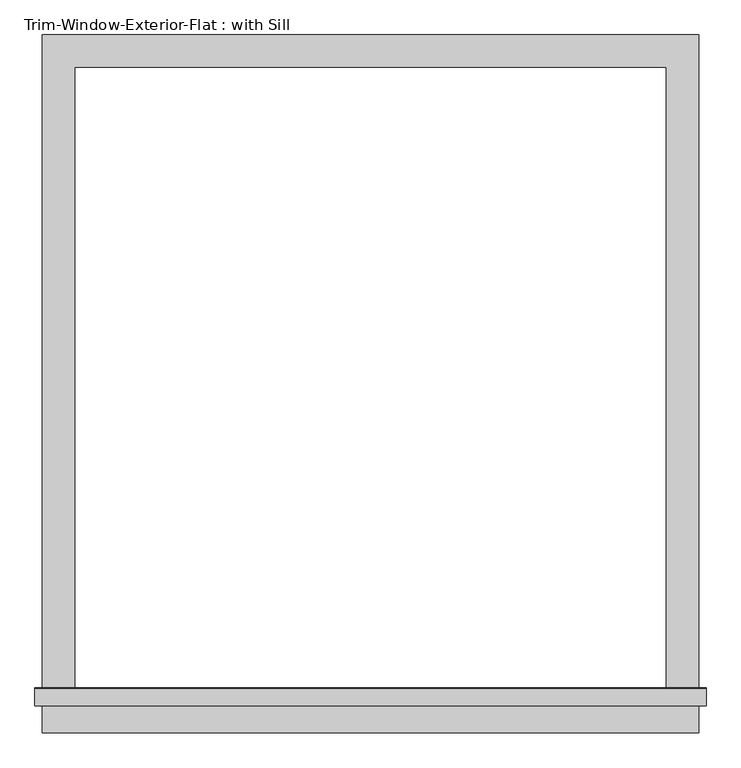
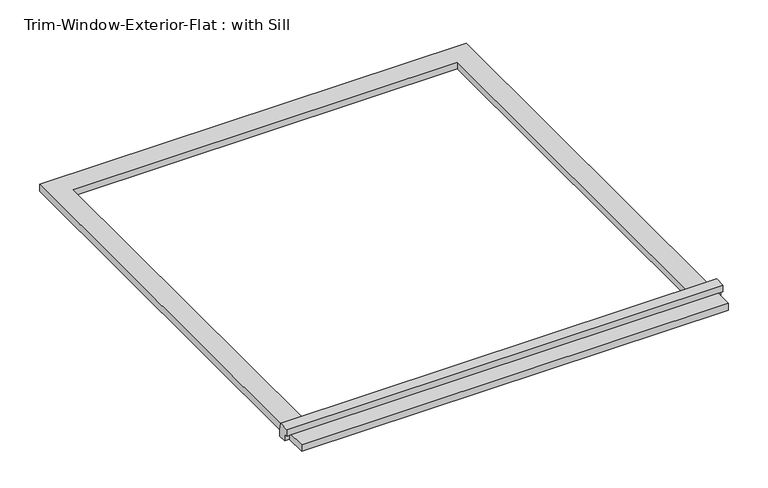
"""IFC4 building model written with IfcOpenShell, lengths in millimetres: proxy geometry, Trim-Window-Exterior-Flat : with Sill."""

from ifc_helpers import new_model, si_unit, frame, origin, origin_with_axes, place, context, project, spatial, polyline, outline, extrude, source, transform, mapped, element, save


def trim_window_exterior_flat_with_sill_d43e16eb(model_context):
    return source(origin(), model_context, "Body", "SweptSolid", [
        extrude(outline(polyline([(577.85, -1114.3823709), (577.85, -1171.5323709), (-577.85, -1171.5323709), (-577.85, -1114.3823709), (577.85, -1114.3823709)])), origin_with_axes(), (0.0, 0.0, 1.0), 19.05),
        extrude(outline(polyline([(-1123.95, 38.1), (-1094.6580645, 38.1), (-1092.2, 19.05), (-1092.2, 0.0), (-1114.3823709, 0.0), (-1114.3823709, 19.05), (-1123.95, 19.05), (-1123.95, 38.1)])), frame((-590.55, 0.0, 0.0), z_axis=(1.0, 0.0, 0.0), x_axis=(0.0, 1.0, 0.0)), (0.0, 0.0, 1.0), 1181.1),
        extrude(outline(polyline([(-577.85, 57.15), (577.85, 57.15), (577.85, -1092.2), (520.7, -1092.2), (520.7, 0.0), (-520.7, 0.0), (-520.7, -1092.2), (-577.85, -1092.2), (-577.85, 57.15)])), origin_with_axes(), (0.0, 0.0, 1.0), 19.05),
    ])


if __name__ == "__main__":
    model = new_model("IFC4")
    model_context = context("Model", 3, world=origin())
    ifc_project = project(units=[si_unit("LENGTHUNIT", "METRE", prefix="MILLI")], contexts=[model_context])
    site = spatial("IfcSite", under=ifc_project)
    building = spatial("IfcBuilding", under=site)
    placement = place(None, origin())
    trim_window_exterior_flat_with_sill_shape = trim_window_exterior_flat_with_sill_d43e16eb(model_context)
    element("IfcBuildingElementProxy", 1, Name="Trim-Window-Exterior-Flat : with Sill", ObjectType="Trim-Window-Exterior-Flat : with Sill", at=placement, inside=building, context=model_context, shape_type="MappedRepresentation", body=[
        mapped(trim_window_exterior_flat_with_sill_shape, transform((0.0, 0.0, 0.0), x_axis=(1.0, 0.0, 0.0), y_axis=(0.0, 1.0, 0.0), z_axis=(0.0, 0.0, 1.0))),
    ])
    save(model, "model.ifc")

# Revit data of these elements
# Type "Trim-Window-Exterior-Flat : with Sill"
#   Trim Width = 0' - 2 1/4"
#   Trim Thickness_Picture Frame = 0' - 1 1/4"
#   Trim Thickness_with Sill = 0' - 0 3/4"
#   Sill Thickness = 0' - 1 1/4"
#   Opening Width [instance default] = 2' - 0"
#   Opening Height [instance default] = 3' - 0"
#   Default Elevation = 4' - 0"
#   Sill = yes
#   Picture Frame = no
#   Trim Material [instance default] = none
# Element 1 (IfcBuildingElementProxy, "Trim-Window-Exterior-Flat : with Sill")
#   Opening Width = 3' - 5"
#   Opening Height = 3' - 7"
#   Trim Material = Clad - White
#   Materials on its faces: "Clad - White"
# Materials
#   "Clad - White": class "Wood", colour RGB 242 242 238, transparency 0, Cost = 0
